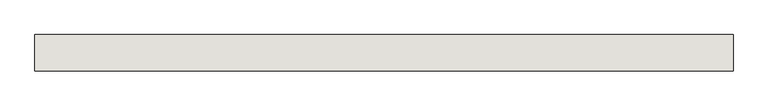
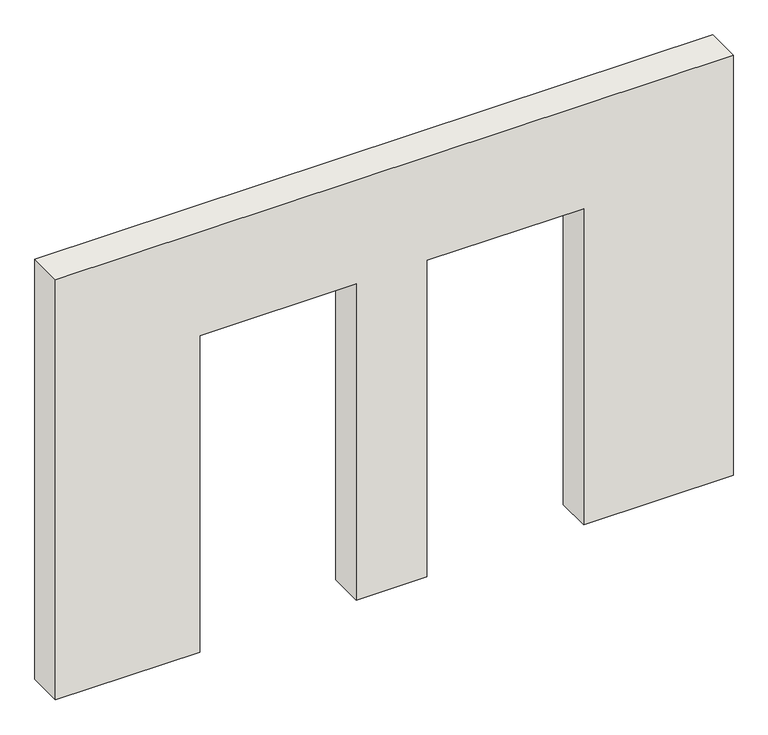
"""IFC4 building model written with IfcOpenShell, lengths in millimetres: wall geometry, Holzwand."""

from ifc_helpers import new_model, si_unit, frame, origin, place, context, project, spatial, polyline, outline, extrude, source, transform, mapped, element, save


def wall_44f19d32(model_context):
    return source(origin(), model_context, "Body", "SweptSolid", [
        extrude(outline(polyline([(0.0, 2100.0), (1890.0, 2100.0), (1890.0, 2985.0), (0.0, 2985.0), (0.0, 3830.0), (2510.0, 3830.0), (2510.0, 0.0), (0.0, 0.0), (0.0, 815.0), (1890.0, 815.0), (1890.0, 1700.0), (0.0, 1700.0), (0.0, 2100.0)])), frame((0.0, 0.0, 0.0), z_axis=(0.0, 1.0, 0.0), x_axis=(0.0, 0.0, 1.0)), (0.0, 0.0, 1.0), 200.0),
    ])


if __name__ == "__main__":
    model = new_model("IFC4")
    model_context = context("Model", 3, world=origin())
    ifc_project = project(units=[si_unit("LENGTHUNIT", "METRE", prefix="MILLI")], contexts=[model_context])
    site = spatial("IfcSite", under=ifc_project)
    building = spatial("IfcBuilding", under=site)
    placement = place(None, origin())
    wall_shape = wall_44f19d32(model_context)
    element("IfcWall", 1, ObjectType="Holzwand", at=placement, inside=building, context=model_context, shape_type="MappedRepresentation", body=[
        mapped(wall_shape, transform((0.0, 0.0, 0.0), x_axis=(1.0, 0.0, 0.0), y_axis=(0.0, 1.0, 0.0), z_axis=(0.0, 0.0, 1.0))),
    ])
    save(model, "model.ifc")

# Revit data of these elements
# Element 1 (IfcWall, "Holzwand")
#   Materials on its faces: "holzschalung"
# Materials
#   "holzschalung": class "Unassigned", colour RGB 128 128 128, transparency 0
